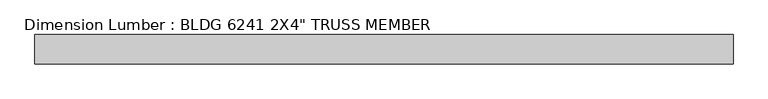
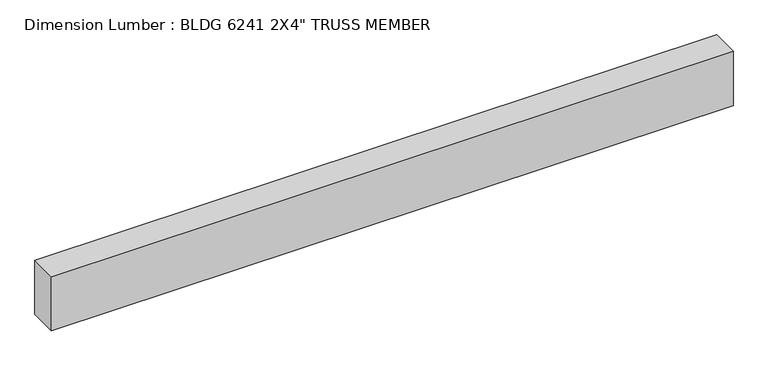
"""IFC4 building model written with IfcOpenShell, lengths in millimetres: beam geometry."""

from ifc_helpers import new_model, si_unit, frame, origin, place, context, project, spatial, polyline, outline, extrude, source, transform, mapped, element, save


def beam_38027485(model_context):
    return source(origin(), model_context, "Body", "SweptSolid", [
        extrude(outline(polyline([(595.8662636, 25.4), (595.8662636, -25.4), (-609.6, -25.4), (-609.6, 25.4), (595.8662636, 25.4)])), frame((0.0, 0.0, -50.8), z_axis=(0.0, 0.0, 1.0), x_axis=(1.0, 0.0, 0.0)), (0.0, 0.0, 1.0), 101.6),
    ])


if __name__ == "__main__":
    model = new_model("IFC4")
    model_context = context("Model", 3, world=origin())
    ifc_project = project(units=[si_unit("LENGTHUNIT", "METRE", prefix="MILLI")], contexts=[model_context])
    site = spatial("IfcSite", under=ifc_project)
    building = spatial("IfcBuilding", under=site)
    placement = place(None, origin())
    beam_shape = beam_38027485(model_context)
    element("IfcBeam", 1, ObjectType="Dimension Lumber : BLDG 6241 2X4\" TRUSS MEMBER", at=placement, inside=building, context=model_context, shape_type="MappedRepresentation", body=[
        mapped(beam_shape, transform((0.0, 0.0, 0.0), x_axis=(1.0, 0.0, 0.0), y_axis=(0.0, 1.0, 0.0), z_axis=(0.0, 0.0, 1.0))),
    ])
    save(model, "model.ifc")

# Revit data of these elements
# Type "Dimension Lumber : BLDG 6241 2X4\" TRUSS MEMBER"
#   Assembly Code = "B10"
#   A = 0.273472 SF
#   Length [instance default] = 5' - 0"
#   b = 0' - 2"
#   d = 0' - 4"
#   Structural Material [instance default] = Softwood, Lumber
# Element 1 (IfcBeam, "Dimension Lumber : BLDG 6241 2X4\" TRUSS MEMBER")
#   Materials on its faces: "Softwood, Lumber"
# Materials
#   "Softwood, Lumber": class "Wood", colour RGB 223 192 134, transparency 0, Description = "Pinus Echinata", Cost = 0
